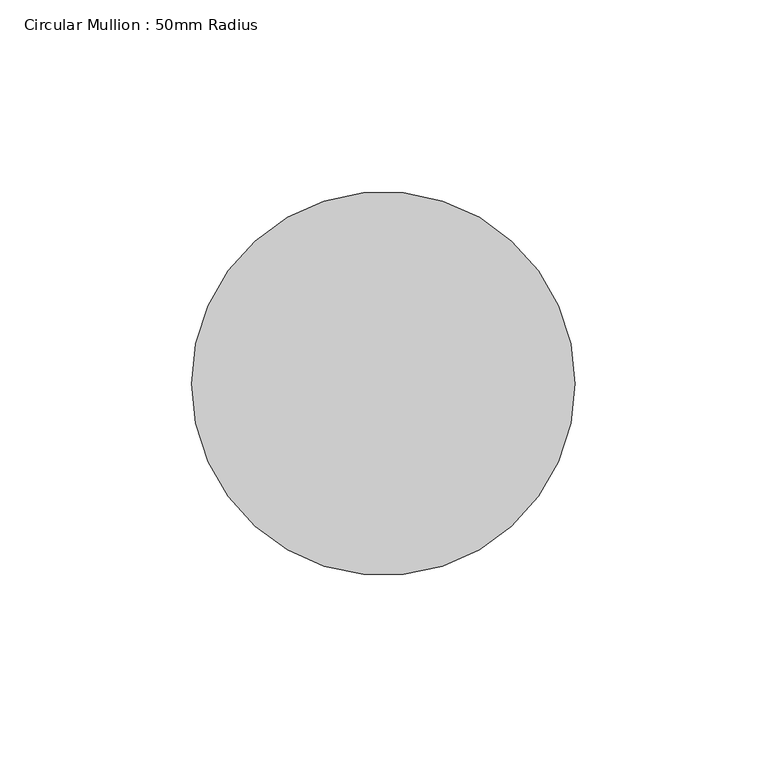
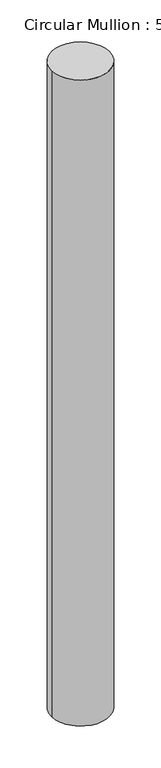
"""IFC4 building model written with IfcOpenShell, lengths in millimetres: member geometry, Circular Mullion : 50mm Radius."""

from ifc_helpers import new_model, si_unit, point, frame, origin, origin_2d, place, context, project, spatial, circle_curve, trimmed, segment, composite_curve, outline, extrude, source, transform, mapped, element, save


def circular_mullion_50mm_radius_75f7242f(model_context):
    return source(origin(), model_context, "Body", "SweptSolid", [
        extrude(outline(composite_curve([segment(trimmed(circle_curve(origin_2d(), 50.0), [point((50.0, 0.0))], [point((-50.0, 0.0))], False, "CARTESIAN"), True, "CONTINUOUS"), segment(trimmed(circle_curve(origin_2d(), 50.0), [point((-50.0, 0.0))], [point((50.0, 0.0))], False, "CARTESIAN"), True, "CONTINUOUS")], self_intersect=False)), frame((0.0, 0.0, -1183.082065), z_axis=(0.0, 0.0, 1.0), x_axis=(1.0, 0.0, 0.0)), (0.0, 0.0, 1.0), 1183.082065),
    ])


if __name__ == "__main__":
    model = new_model("IFC4")
    model_context = context("Model", 3, world=origin())
    ifc_project = project(units=[si_unit("LENGTHUNIT", "METRE", prefix="MILLI")], contexts=[model_context])
    site = spatial("IfcSite", under=ifc_project)
    building = spatial("IfcBuilding", under=site)
    placement = place(None, origin())
    circular_mullion_50mm_radius_shape = circular_mullion_50mm_radius_75f7242f(model_context)
    element("IfcMember", 1, ObjectType="Circular Mullion : 50mm Radius", at=placement, inside=building, context=model_context, shape_type="MappedRepresentation", body=[
        mapped(circular_mullion_50mm_radius_shape, transform((0.0, 0.0, 0.0), x_axis=(1.0, 0.0, 0.0), y_axis=(0.0, 1.0, 0.0), z_axis=(0.0, 0.0, 1.0))),
    ])
    save(model, "model.ifc")

# Revit data of these elements
# Type "Circular Mullion : 50mm Radius"
#   built-in parameter 1007350 = 0.164042 (stored number, unit not read)
# Element 1 (IfcMember, "Circular Mullion : 50mm Radius")
#   Materials on its faces: "Aluminium"
# Materials
#   "Aluminium": class "Metal", colour RGB 247 247 247, transparency 0, Description = "Aluminium 6061", Cost = 0
